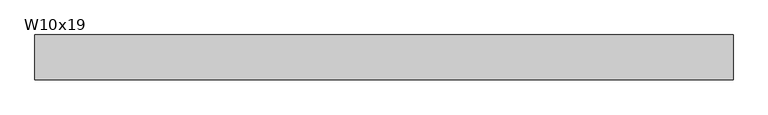
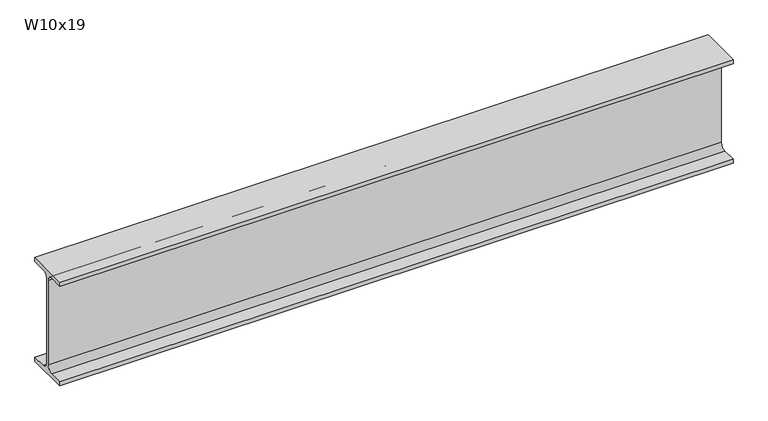
"""IFC4 building model written with IfcOpenShell, lengths in millimetres: beam geometry, RME W-Wide Flange : W10x19."""

from ifc_helpers import new_model, si_unit, point, frame, frame_2d, origin, place, context, project, spatial, polyline, circle_curve, trimmed, segment, composite_curve, outline, extrude, source, transform, mapped, element, save


def w10x19_6aab4d3a(model_context):
    return source(origin(), model_context, "Body", "SweptSolid", [
        extrude(outline(composite_curve([segment(polyline([(51.054, -119.507), (51.054, -129.54), (-51.054, -129.54), (-51.054, -119.507), (-16.9545, -119.507)]), True, "CONTINUOUS"), segment(trimmed(circle_curve(frame_2d((-16.9545, -105.7275)), 13.7795), [point((-16.9545, -119.507))], [point((-3.175, -105.7275))], True, "CARTESIAN"), True, "CONTINUOUS"), segment(polyline([(-3.175, -105.7275), (-3.175, 105.7275)]), True, "CONTINUOUS"), segment(trimmed(circle_curve(frame_2d((-16.9545, 105.7275)), 13.7795), [point((-3.175, 105.7275))], [point((-16.9545, 119.507))], True, "CARTESIAN"), True, "CONTINUOUS"), segment(polyline([(-16.9545, 119.507), (-51.054, 119.507), (-51.054, 129.54), (51.054, 129.54), (51.054, 119.507), (16.9545, 119.507)]), True, "CONTINUOUS"), segment(trimmed(circle_curve(frame_2d((16.9545, 105.7275)), 13.7795), [point((16.9545, 119.507))], [point((3.175, 105.7275))], True, "CARTESIAN"), True, "CONTINUOUS"), segment(polyline([(3.175, 105.7275), (3.175, -105.7275)]), True, "CONTINUOUS"), segment(trimmed(circle_curve(frame_2d((16.9545, -105.7275)), 13.7795), [point((3.175, -105.7275))], [point((16.9545, -119.507))], True, "CARTESIAN"), True, "CONTINUOUS"), segment(polyline([(16.9545, -119.507), (51.054, -119.507)]), True, "CONTINUOUS")], self_intersect=False)), frame((-763.0341711, 0.0, 0.0), z_axis=(1.0, 0.0, 0.0), x_axis=(0.0, 1.0, 0.0)), (0.0, 0.0, 1.0), 1589.8223422),
    ])


if __name__ == "__main__":
    model = new_model("IFC4")
    model_context = context("Model", 3, world=origin())
    ifc_project = project(units=[si_unit("LENGTHUNIT", "METRE", prefix="MILLI")], contexts=[model_context])
    site = spatial("IfcSite", under=ifc_project)
    building = spatial("IfcBuilding", under=site)
    placement = place(None, origin())
    w10x19_shape = w10x19_6aab4d3a(model_context)
    element("IfcBeam", 1, ObjectType="RME W-Wide Flange : W10x19", at=placement, inside=building, context=model_context, shape_type="MappedRepresentation", body=[
        mapped(w10x19_shape, transform((0.0, 0.0, 0.0), x_axis=(1.0, 0.0, 0.0), y_axis=(0.0, 1.0, 0.0), z_axis=(0.0, 0.0, 1.0))),
    ])
    save(model, "model.ifc")

# Revit data of these elements
# Type "RME W-Wide Flange : W10x19"
#   WELD P [instance default] = ""
#   WELD LE [instance default] = ""
#   WELD D [instance default] = ""
#   TOP SECTION SIZE [instance default] = ""
#   TOP SECTION LENGTH [instance default] = ""
#   REMARKS [instance default] = ""
#   REINF TYPE [instance default] = ""
#   Nominal Size = "W24"
#   End Bearing Capacity [instance default] = ""
#   BOT SECTION SIZE [instance default] = ""
#   BOT SECTION LENGTH [instance default] = ""
#   Assembly Code = "B10"
#   W = 19
#   Start Extension Calculation [instance default] = 10' - 0"
#   Start Extension [instance default] = -0' - 0 1/2"
#   End Extension Calculation [instance default] = 10' - 0"
#   End Extension [instance default] = -0' - 0 1/2"
#   Length [instance default] = 5' - 0"
#   bf = 0' - 4.02"
#   d = 0' - 10.2"
#   k = 0' - 0 15/16"
#   k2 = 0' - 0.5425"
#   tf = 0' - 0.395"
#   tw = 0' - 0 1/4"
#   A = 0.0390278 SF
#   Structural Material [instance default] = Metal - Steel - ASTM A992
# Element 1 (IfcBeam, "RME W-Wide Flange : W10x19")
#   Length = 5' - 5.10143"
#   Materials on its faces: "Metal - Steel - ASTM A992"
# Materials
#   "Metal - Steel - ASTM A992": class "Metal", colour RGB 255 128 0, transparency 0
